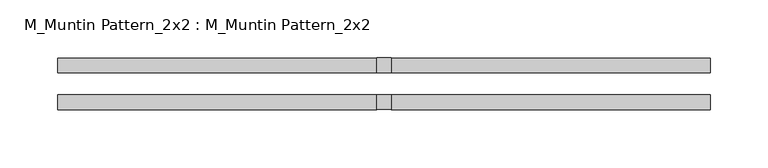
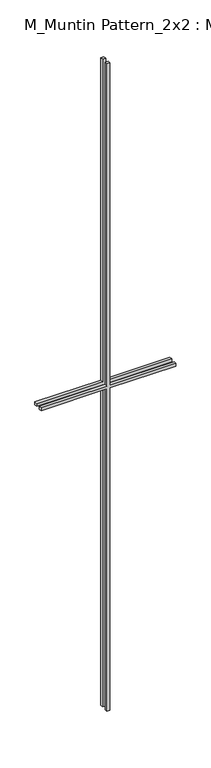
"""IFC4 building model written with IfcOpenShell, lengths in millimetres: proxy geometry, M_Muntin Pattern_2x2 : M_Muntin Pattern_2x2."""

from ifc_helpers import new_model, si_unit, frame, origin, place, context, project, spatial, polyline, outline, extrude, source, transform, mapped, element, save


def m_muntin_pattern_2x2_m_muntin_pattern_2x2_57defa01(model_context):
    return source(origin(), model_context, "Body", "SweptSolid", [
        extrude(outline(polyline([(1436.5, -6.35), (1436.5, -281.7375), (1423.8, -281.7375), (1423.8, -6.35), (0.0, -6.35), (0.0, 6.35), (1423.8, 6.35), (1423.8, 281.7375), (1436.5, 281.7375), (1436.5, 6.35), (2860.3, 6.35), (2860.3, -6.35), (1436.5, -6.35)])), frame((0.0, -22.225, 0.0), z_axis=(0.0, 1.0, 0.0), x_axis=(0.0, 0.0, 1.0)), (0.0, 0.0, 1.0), 12.7),
        extrude(outline(polyline([(1436.5, -6.35), (1436.5, -281.7375), (1423.8, -281.7375), (1423.8, -6.35), (0.0, -6.35), (0.0, 6.35), (1423.8, 6.35), (1423.8, 281.7375), (1436.5, 281.7375), (1436.5, 6.35), (2860.3, 6.35), (2860.3, -6.35), (1436.5, -6.35)])), frame((0.0, 9.525, 0.0), z_axis=(0.0, 1.0, 0.0), x_axis=(0.0, 0.0, 1.0)), (0.0, 0.0, 1.0), 12.7),
    ])


if __name__ == "__main__":
    model = new_model("IFC4")
    model_context = context("Model", 3, world=origin())
    ifc_project = project(units=[si_unit("LENGTHUNIT", "METRE", prefix="MILLI")], contexts=[model_context])
    site = spatial("IfcSite", under=ifc_project)
    building = spatial("IfcBuilding", under=site)
    placement = place(None, origin())
    m_muntin_pattern_2x2_m_muntin_pattern_2x2_shape = m_muntin_pattern_2x2_m_muntin_pattern_2x2_57defa01(model_context)
    element("IfcBuildingElementProxy", 1, Name="M_Muntin Pattern_2x2 : M_Muntin Pattern_2x2", ObjectType="M_Muntin Pattern_2x2 : M_Muntin Pattern_2x2", at=placement, inside=building, context=model_context, shape_type="MappedRepresentation", body=[
        mapped(m_muntin_pattern_2x2_m_muntin_pattern_2x2_shape, transform((0.0, 0.0, 0.0), x_axis=(1.0, 0.0, 0.0), y_axis=(0.0, 1.0, 0.0), z_axis=(0.0, 0.0, 1.0))),
    ])
    save(model, "model.ifc")

# Revit data of these elements
# Type "M_Muntin Pattern_2x2 : M_Muntin Pattern_2x2"
#   Width [instance default] = 1200 mm
#   Thickness = 12.7 mm
#   Height [instance default] = 1200 mm
#   Distance = 19.05 mm
#   Interior Material [instance default] = none
#   Exterior Material [instance default] = none
#   Default Elevation = 0
# Element 1 (IfcBuildingElementProxy, "M_Muntin Pattern_2x2 : M_Muntin Pattern_2x2")
#   Width = 563.475 mm
#   Height = 2860.3 mm
#   Interior Material = Wood - Stained
#   Exterior Material = Clad - White
#   Materials on its faces: "Clad - White", "Wood - Stained"
# Materials
#   "Clad - White": class "Wood", colour RGB 245 245 243, transparency 0, Cost = 0
#   "Wood - Stained": class "Wood", colour RGB 173 132 96, transparency 0, Cost = 0
